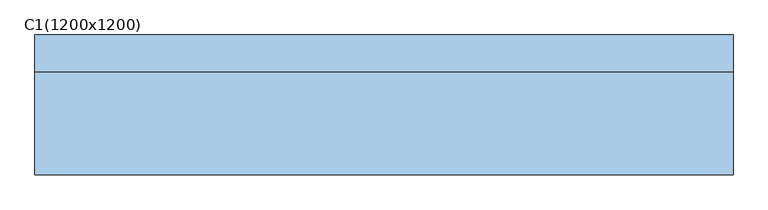
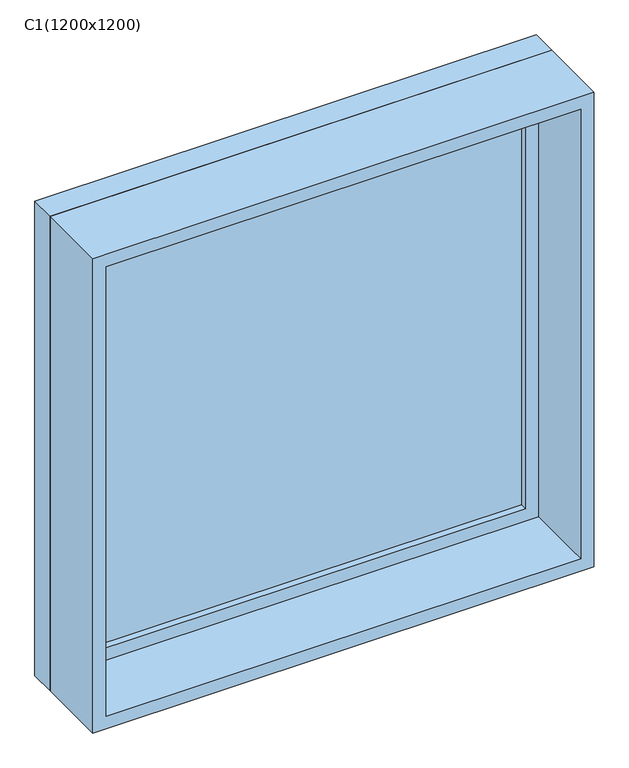
"""IFC4 building model written with IfcOpenShell, lengths in millimetres: window geometry, 固定窗 : C1(1200x1200)."""

from ifc_helpers import new_model, si_unit, frame, origin, place, context, project, spatial, polyline, outline, extrude, source, transform, mapped, element, save


def c1_1200x1200_024adce4(model_context):
    return source(origin(), model_context, "Body", "SweptSolid", [
        extrude(outline(polyline([(498.4, 71.425), (-574.6, 71.425), (-574.6, 84.125), (498.4, 84.125), (498.4, 71.425)])), frame((0.0, 0.0, 963.5), z_axis=(0.0, 0.0, 1.0), x_axis=(1.0, 0.0, 0.0)), (0.0, 0.0, 1.0), 1073.0),
        extrude(outline(polyline([(2080.95, -619.05), (919.05, -619.05), (919.05, 542.85), (2080.95, 542.85), (2080.95, -619.05)]), holes=[polyline([(2036.5, -574.6), (2036.5, 498.4), (963.5, 498.4), (963.5, -574.6), (2036.5, -574.6)])]), frame((0.0, 55.55, 0.0), z_axis=(0.0, 1.0, 0.0), x_axis=(0.0, 0.0, 1.0)), (0.0, 0.0, 1.0), 44.45),
        extrude(outline(polyline([(2100.0, -638.1), (900.0, -638.1), (900.0, 561.9), (2100.0, 561.9), (2100.0, -638.1)]), holes=[polyline([(2068.25, -606.35), (2068.25, 530.15), (931.75, 530.15), (931.75, -606.35), (2068.25, -606.35)])]), frame((0.0, -120.0, 0.0), z_axis=(0.0, 1.0, 0.0), x_axis=(0.0, 0.0, 1.0)), (0.0, 0.0, 1.0), 175.55),
        extrude(outline(polyline([(2100.0, 561.9), (2100.0, -638.1), (900.0, -638.1), (900.0, 561.9), (2100.0, 561.9)]), holes=[polyline([(2080.95, 542.85), (919.05, 542.85), (919.05, -619.05), (2080.95, -619.05), (2080.95, 542.85)])]), frame((0.0, 55.55, 0.0), z_axis=(0.0, 1.0, 0.0), x_axis=(0.0, 0.0, 1.0)), (0.0, 0.0, 1.0), 64.45),
    ])


if __name__ == "__main__":
    model = new_model("IFC4")
    model_context = context("Model", 3, world=origin())
    ifc_project = project(units=[si_unit("LENGTHUNIT", "METRE", prefix="MILLI")], contexts=[model_context])
    site = spatial("IfcSite", under=ifc_project)
    building = spatial("IfcBuilding", under=site)
    placement = place(None, origin())
    c1_1200x1200_shape = c1_1200x1200_024adce4(model_context)
    element("IfcWindow", 1, ObjectType="固定窗 : C1(1200x1200)", at=placement, inside=building, context=model_context, shape_type="MappedRepresentation", body=[
        mapped(c1_1200x1200_shape, transform((0.0, 0.0, 0.0), x_axis=(1.0, 0.0, 0.0), y_axis=(0.0, 1.0, 0.0), z_axis=(0.0, 0.0, 1.0))),
    ])
    save(model, "model.ifc")

# Revit data of these elements
# Type "固定窗 : C1(1200x1200)"
#   Type Mark = "C1518"
#   Construction Type Id = "SGL"
#   Analytic Construction = "大型单层玻璃窗"
#   Visual Light Transmittance = 0.9
#   Solar Heat Gain Coefficient = 0.86
#   Rough Width = 1200 mm
#   Rough Height = 1200 mm
#   Heat Transfer Coefficient (U) = 5.5617 W/(m²·K)
#   Height = 1200 mm
#   默认窗台高度 = 900 mm
#   Width = 1200 mm
#   窗嵌入 = 20 mm
#   高窗平面 [instance default] = no
#   通用窗平面 [instance default] = yes
#   玻璃 = none
#   框架材质 = none
#   Wall Closure = (empty or 0)
# Element 1 (IfcWindow, "固定窗 : C1(1200x1200)")
#   Materials on its faces: "玻璃"
# Materials
#   "玻璃": class "玻璃", colour RGB 0 128 192, transparency 0.9, Description = "钠钙玻璃", Cost = 0
